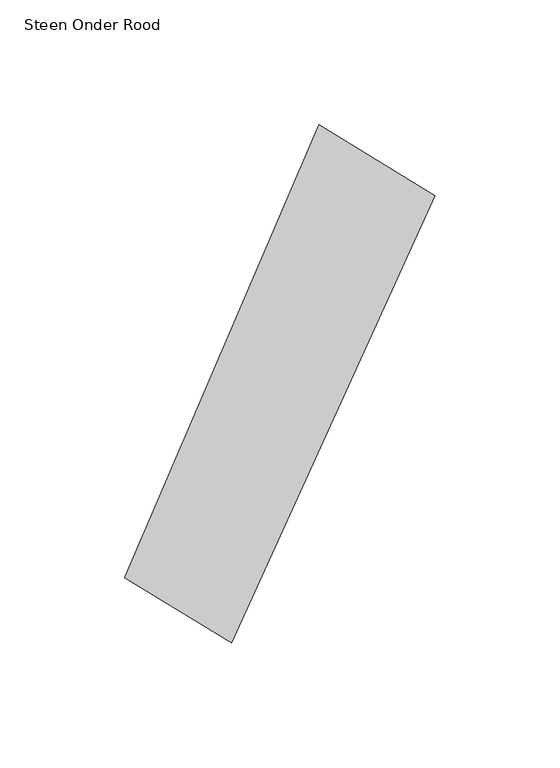
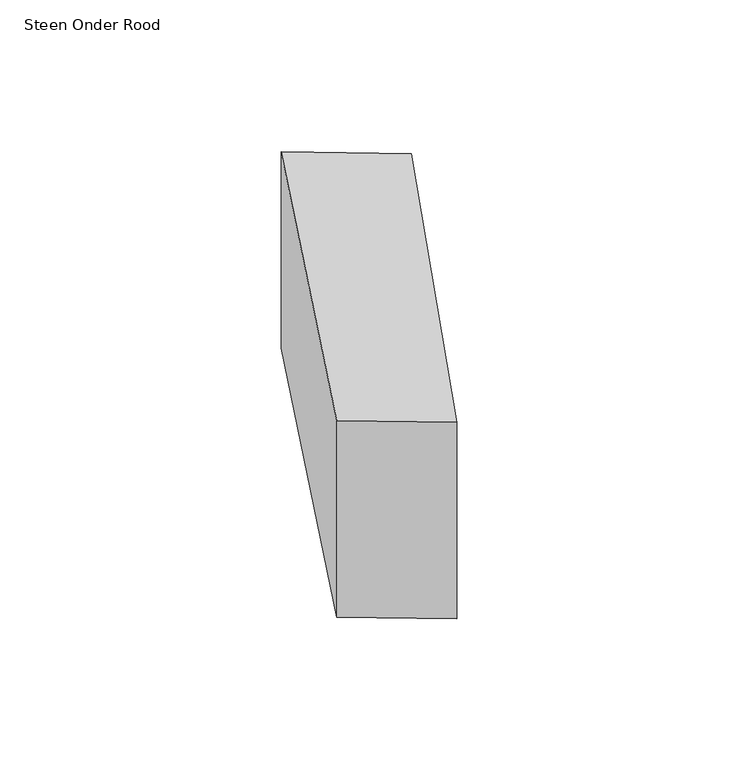
"""IFC4 building model written with IfcOpenShell, lengths in millimetres: proxy geometry, 00_GMA_steen_versie_4 : Steen Onder Rood."""

from ifc_helpers import new_model, si_unit, origin, origin_with_axes, place, context, project, spatial, polyline, outline, extrude, source, transform, mapped, element, save


def steen_onder_rood_4cd60e78(model_context):
    return source(origin(), model_context, "Body", "SweptSolid", [
        extrude(outline(polyline([(140.955132, 158.3459997), (59.5486665, -20.4865271), (16.8910304, 5.5965341), (94.6043783, 186.7015026), (140.955132, 158.3459997)])), origin_with_axes(), (0.0, 0.0, 1.0), 100.0),
    ])


if __name__ == "__main__":
    model = new_model("IFC4")
    model_context = context("Model", 3, world=origin())
    ifc_project = project(units=[si_unit("LENGTHUNIT", "METRE", prefix="MILLI")], contexts=[model_context])
    site = spatial("IfcSite", under=ifc_project)
    building = spatial("IfcBuilding", under=site)
    placement = place(None, origin())
    steen_onder_rood_shape = steen_onder_rood_4cd60e78(model_context)
    element("IfcBuildingElementProxy", 1, Name="00_GMA_steen_versie_4 : Steen Onder Rood", ObjectType="00_GMA_steen_versie_4 : Steen Onder Rood", at=placement, inside=building, context=model_context, shape_type="MappedRepresentation", body=[
        mapped(steen_onder_rood_shape, transform((0.0, 0.0, 0.0), x_axis=(1.0, 0.0, 0.0), y_axis=(0.0, 1.0, 0.0), z_axis=(0.0, 0.0, 1.0))),
    ])
    save(model, "model.ifc")

# Revit data of these elements
# Type "00_GMA_steen_versie_4 : Steen Onder Rood"
#   StootVoegHalfBoven [instance default] = 5 mm
#   StootVoegHalf [instance default] = 5 mm
#   StootVoegBreedteOnder = 10 mm
#   StootVoegBreedteBoven = 10 mm
#   Steendikte = 100 mm
#   LintVoegOnderHalf = 0 mm
#   LintVoegOnder = 0 mm
#   LintVoegBovenHalf = 5 mm
#   LintVoegBoven = 10 mm
#   materiaal = 21_steen_rood
#   MateriaalVoeg = none
#   Default Elevation = 0
# Element 1 (IfcBuildingElementProxy, "00_GMA_steen_versie_4 : Steen Onder Rood")
#   Materials on its faces: "21_steen_rood"
# Materials
#   "21_steen_rood": class "Unassigned", colour RGB 213 111 43, transparency 0, Cost = 0
